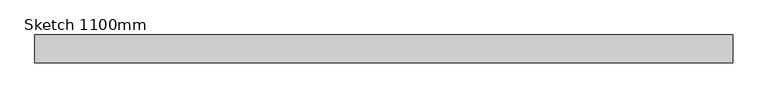
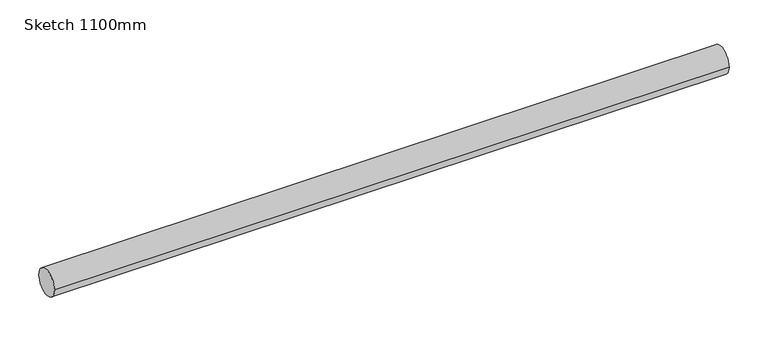
"""IFC4 building model written with IfcOpenShell, lengths in millimetres: railing geometry, Sketch 1100mm."""

from ifc_helpers import new_model, si_unit, point, frame, frame_2d, origin, place, context, project, spatial, circle_curve, trimmed, segment, composite_curve, outline, extrude, source, transform, mapped, element, save


def sketch_1100mm_82aaa055(model_context):
    return source(origin(), model_context, "Body", "SweptSolid", [
        extrude(outline(composite_curve([segment(trimmed(circle_curve(frame_2d((5300.0, 7480.0)), 20.0), [point((5280.0, 7480.0))], [point((5320.0, 7480.0))], False, "CARTESIAN"), True, "CONTINUOUS"), segment(trimmed(circle_curve(frame_2d((5300.0, 7480.0)), 20.0), [point((5320.0, 7480.0))], [point((5280.0, 7480.0))], False, "CARTESIAN"), True, "CONTINUOUS")], self_intersect=False)), frame((7925.0, 0.0, 0.0), z_axis=(1.0, 0.0, 0.0), x_axis=(0.0, 1.0, 0.0)), (0.0, 0.0, 1.0), 1000.0),
    ])


if __name__ == "__main__":
    model = new_model("IFC4")
    model_context = context("Model", 3, world=origin())
    ifc_project = project(units=[si_unit("LENGTHUNIT", "METRE", prefix="MILLI")], contexts=[model_context])
    site = spatial("IfcSite", under=ifc_project)
    building = spatial("IfcBuilding", under=site)
    placement = place(None, origin())
    sketch_1100mm_shape = sketch_1100mm_82aaa055(model_context)
    element("IfcRailing", 1, ObjectType="Sketch 1100mm", at=placement, inside=building, context=model_context, shape_type="MappedRepresentation", body=[
        mapped(sketch_1100mm_shape, transform((0.0, 0.0, 0.0), x_axis=(1.0, 0.0, 0.0), y_axis=(0.0, 1.0, 0.0), z_axis=(0.0, 0.0, 1.0))),
    ])
    save(model, "model.ifc")

# Revit data of these elements
# Element 1 (IfcRailing, "Sketch 1100mm")
#   Materials on its faces: "Default Railings (Interior/Exterior)"
# Materials
#   "Default Railings (Interior/Exterior)": class "Generic", colour RGB 205 205 205, transparency 0, Description = "Udefineret gelænder materiale", Cost = 0
